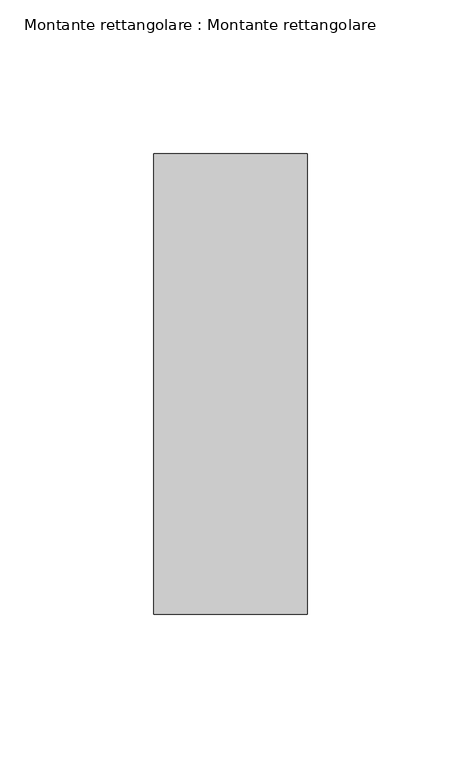
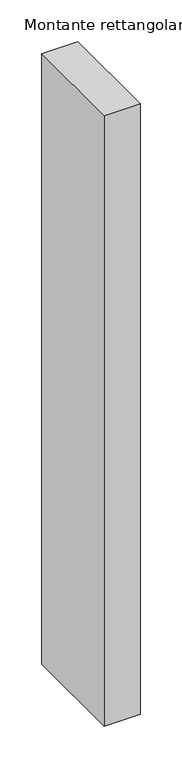
"""IFC4 building model written with IfcOpenShell, lengths in millimetres: member geometry, Montante rettangolare : Montante rettangolare."""

from ifc_helpers import new_model, si_unit, frame, origin, place, context, project, spatial, polyline, outline, extrude, source, transform, mapped, element, save


def montante_rettangolare_montante_rettangolare_8bb159a6(model_context):
    return source(origin(), model_context, "Body", "SweptSolid", [
        extrude(outline(polyline([(25.0, 75.0), (25.0, -75.0), (-25.0, -75.0), (-25.0, 75.0), (25.0, 75.0)])), frame((0.0, 0.0, -895.0), z_axis=(0.0, 0.0, 1.0), x_axis=(1.0, 0.0, 0.0)), (0.0, 0.0, 1.0), 895.0),
    ])


if __name__ == "__main__":
    model = new_model("IFC4")
    model_context = context("Model", 3, world=origin())
    ifc_project = project(units=[si_unit("LENGTHUNIT", "METRE", prefix="MILLI")], contexts=[model_context])
    site = spatial("IfcSite", under=ifc_project)
    building = spatial("IfcBuilding", under=site)
    placement = place(None, origin())
    montante_rettangolare_montante_rettangolare_shape = montante_rettangolare_montante_rettangolare_8bb159a6(model_context)
    element("IfcMember", 1, ObjectType="Montante rettangolare : Montante rettangolare", at=placement, inside=building, context=model_context, shape_type="MappedRepresentation", body=[
        mapped(montante_rettangolare_montante_rettangolare_shape, transform((0.0, 0.0, 0.0), x_axis=(1.0, 0.0, 0.0), y_axis=(0.0, 1.0, 0.0), z_axis=(0.0, 0.0, 1.0))),
    ])
    save(model, "model.ifc")

# Revit data of these elements
# Type "Montante rettangolare : Montante rettangolare"
#   built-in parameter 1007304 = 0.492126 (stored number, unit not read)
#   built-in parameter 1007301 = 0.082021 (stored number, unit not read)
#   built-in parameter 1007300 = 0.082021 (stored number, unit not read)
# Element 1 (IfcMember, "Montante rettangolare : Montante rettangolare")
#   Materials on its faces: "Acciaio"
# Materials
#   "Acciaio": class "Metallo", colour RGB 247 247 247, transparency 0, Description = "Acciaio, finitura zigrinata", Cost = 0
